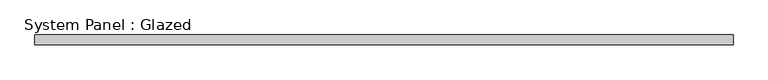
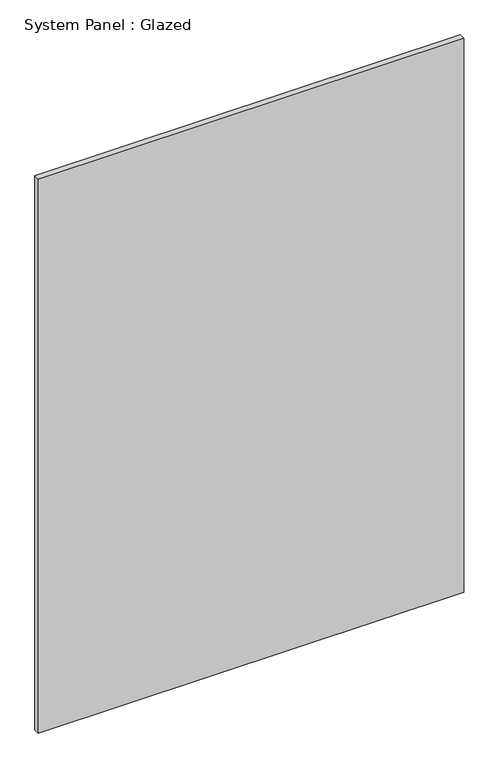
"""IFC4 building model written with IfcOpenShell, lengths in millimetres: plate geometry, System Panel : Glazed."""

from ifc_helpers import new_model, si_unit, origin, origin_with_axes, place, context, project, spatial, polyline, outline, extrude, source, transform, mapped, element, save


def system_panel_glazed_55ebe308(model_context):
    return source(origin(), model_context, "Body", "SweptSolid", [
        extrude(outline(polyline([(890.0, -49.5), (-890.0, -49.5), (-890.0, -24.5), (890.0, -24.5), (890.0, -49.5)])), origin_with_axes(), (0.0, 0.0, 1.0), 2450.0),
    ])


if __name__ == "__main__":
    model = new_model("IFC4")
    model_context = context("Model", 3, world=origin())
    ifc_project = project(units=[si_unit("LENGTHUNIT", "METRE", prefix="MILLI")], contexts=[model_context])
    site = spatial("IfcSite", under=ifc_project)
    building = spatial("IfcBuilding", under=site)
    placement = place(None, origin())
    system_panel_glazed_shape = system_panel_glazed_55ebe308(model_context)
    element("IfcPlate", 1, ObjectType="System Panel : Glazed", at=placement, inside=building, context=model_context, shape_type="MappedRepresentation", body=[
        mapped(system_panel_glazed_shape, transform((0.0, 0.0, 0.0), x_axis=(1.0, 0.0, 0.0), y_axis=(0.0, 1.0, 0.0), z_axis=(0.0, 0.0, 1.0))),
    ])
    save(model, "model.ifc")

# Revit data of these elements
# Type "System Panel : Glazed"
#   Keynote = "H11"
#   Construction Type Id = "GSP4R"
#   Analytic Construction = "1/8 in Pilkington single glazing"
#   Visual Light Transmittance = 0.9
#   Solar Heat Gain Coefficient = 0.86
#   Heat Transfer Coefficient (U) = 6.7069 W/(m²·K)
# Element 1 (IfcPlate, "System Panel : Glazed")
#   Materials on its faces: "Glass"
# Materials
#   "Glass": class "Glass", colour RGB 0 128 192, transparency 0.9, Description = "Soda Lime Glass", Cost = 0
